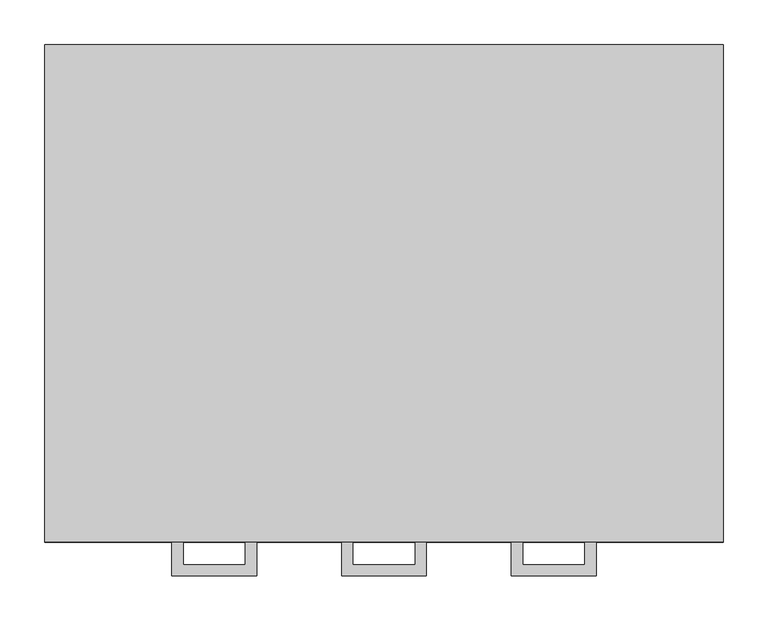
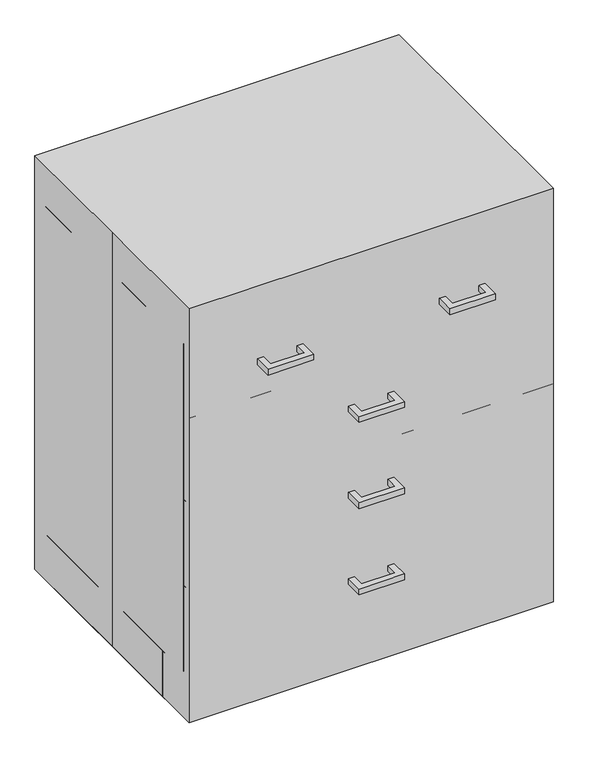
"""IFC4 building model written with IfcOpenShell, lengths in millimetres: proxy geometry, C03H0 - Cabinet, U-C-B, 2 Half DR, 3 DR, 36x30x22 : C03H0 - Cabinet, U-C-B, 2 Half DR, 3 DR, 36x30x22."""

from ifc_helpers import new_model, si_unit, frame, origin, origin_with_axes, place, context, project, spatial, polyline, outline, extrude, source, transform, mapped, element, save


def specialty_equipment_9ec7cdb3(model_context):
    return source(origin(), model_context, "Body", "SweptSolid", [
        extrude(outline(polyline([(-47.625, -317.5), (-47.625, -279.4), (-34.9409299, -279.4), (-34.9409299, -304.8159299), (34.9409299, -304.8159299), (34.9409299, -279.4), (47.625, -279.4), (47.625, -317.5), (-47.625, -317.5)])), frame((0.0, 0.0, 188.8962383), z_axis=(0.0, 0.0, 1.0), x_axis=(1.0, 0.0, 0.0)), (0.0, 0.0, 1.0), 12.7),
        extrude(outline(polyline([(-47.625, -317.5), (-47.625, -279.4), (-34.9409299, -279.4), (-34.9409299, -304.8159299), (34.9409299, -304.8159299), (34.9409299, -279.4), (47.625, -279.4), (47.625, -317.5), (-47.625, -317.5)])), frame((0.0, 0.0, 379.3962383), z_axis=(0.0, 0.0, 1.0), x_axis=(1.0, 0.0, 0.0)), (0.0, 0.0, 1.0), 12.7),
        extrude(outline(polyline([(-47.625, -317.5), (-47.625, -279.4), (-34.9409299, -279.4), (-34.9409299, -304.8159299), (34.9409299, -304.8159299), (34.9409299, -279.4), (47.625, -279.4), (47.625, -317.5), (-47.625, -317.5)])), frame((0.0, 0.0, 569.8962383), z_axis=(0.0, 0.0, 1.0), x_axis=(1.0, 0.0, 0.0)), (0.0, 0.0, 1.0), 12.7),
        extrude(outline(polyline([(-238.125, -317.5), (-238.125, -279.4), (-225.4409299, -279.4), (-225.4409299, -304.8159299), (-155.5590701, -304.8159299), (-155.5590701, -279.4), (-142.875, -279.4), (-142.875, -317.5), (-238.125, -317.5)])), frame((0.0, 0.0, 741.3462383), z_axis=(0.0, 0.0, 1.0), x_axis=(1.0, 0.0, 0.0)), (0.0, 0.0, 1.0), 12.7),
        extrude(outline(polyline([(238.125, -317.5), (142.875, -317.5), (142.875, -279.4), (155.5590701, -279.4), (155.5590701, -304.8159299), (225.4409299, -304.8159299), (225.4409299, -279.4), (238.125, -279.4), (238.125, -317.5)])), frame((0.0, 0.0, 741.3462383), z_axis=(0.0, 0.0, 1.0), x_axis=(1.0, 0.0, 0.0)), (0.0, 0.0, 1.0), 12.7),
        extrude(outline(polyline([(-381.0, 279.4), (381.0, 279.4), (381.0, -279.4), (-381.0, -279.4), (-381.0, 0.0), (-381.0, 279.4)])), origin_with_axes(), (0.0, 0.0, 1.0), 914.4),
        extrude(outline(polyline([(381.0, -279.4), (-381.0, -279.4), (-381.0, -260.35), (381.0, -260.35), (381.0, -279.4)])), frame((0.0, 0.0, 101.5674767), z_axis=(0.0, 0.0, 1.0), x_axis=(1.0, 0.0, 0.0)), (0.0, 0.0, 1.0), 190.5),
        extrude(outline(polyline([(381.0, -279.4), (-381.0, -279.4), (-381.0, -260.35), (381.0, -260.35), (381.0, -279.4)])), frame((0.0, 0.0, 292.0674767), z_axis=(0.0, 0.0, 1.0), x_axis=(1.0, 0.0, 0.0)), (0.0, 0.0, 1.0), 190.5),
        extrude(outline(polyline([(381.0, -279.4), (-381.0, -279.4), (-381.0, -260.35), (381.0, -260.35), (381.0, -279.4)])), frame((0.0, 0.0, 482.5674767), z_axis=(0.0, 0.0, 1.0), x_axis=(1.0, 0.0, 0.0)), (0.0, 0.0, 1.0), 190.5),
        extrude(outline(polyline([(381.0, -279.4), (0.0, -279.4), (0.0, -260.35), (381.0, -260.35), (381.0, -279.4)])), frame((0.0, 0.0, 673.0674767), z_axis=(0.0, 0.0, 1.0), x_axis=(1.0, 0.0, 0.0)), (0.0, 0.0, 1.0), 152.4),
        extrude(outline(polyline([(0.0, -279.4), (-381.0, -279.4), (-381.0, -260.35), (0.0, -260.35), (0.0, -279.4)])), frame((0.0, 0.0, 673.0674767), z_axis=(0.0, 0.0, 1.0), x_axis=(1.0, 0.0, 0.0)), (0.0, 0.0, 1.0), 152.4),
        extrude(outline(polyline([(-381.0, -260.35), (-381.0, 279.4), (-361.95, 279.4), (-361.95, -260.35), (-381.0, -260.35)])), frame((0.0, 0.0, 101.6), z_axis=(0.0, 0.0, 1.0), x_axis=(1.0, 0.0, 0.0)), (0.0, 0.0, 1.0), 723.8674767),
        extrude(outline(polyline([(361.95, -260.35), (361.95, 279.4), (381.0, 279.4), (381.0, -260.35), (361.95, -260.35)])), frame((0.0, 0.0, 101.6), z_axis=(0.0, 0.0, 1.0), x_axis=(1.0, 0.0, 0.0)), (0.0, 0.0, 1.0), 723.8674767),
        extrude(outline(polyline([(381.0, -203.2), (-381.0, -203.2), (-381.0, -184.15), (381.0, -184.15), (381.0, -203.2)])), origin_with_axes(), (0.0, 0.0, 1.0), 101.6),
        extrude(outline(polyline([(-381.0, -184.15), (-381.0, 279.4), (-361.95, 279.4), (-361.95, -184.15), (-381.0, -184.15)])), origin_with_axes(), (0.0, 0.0, 1.0), 101.6),
        extrude(outline(polyline([(361.95, -184.15), (361.95, 279.4), (381.0, 279.4), (381.0, -184.15), (361.95, -184.15)])), origin_with_axes(), (0.0, 0.0, 1.0), 101.6),
        extrude(outline(polyline([(381.0, 260.35), (-381.0, 260.35), (-381.0, 279.4), (381.0, 279.4), (381.0, 260.35)])), origin_with_axes(), (0.0, 0.0, 1.0), 101.6),
        extrude(outline(polyline([(361.95, 260.35), (361.95, -260.35), (-361.95, -260.35), (-361.95, 260.35), (361.95, 260.35)])), frame((0.0, 0.0, 101.6), z_axis=(0.0, 0.0, 1.0), x_axis=(1.0, 0.0, 0.0)), (0.0, 0.0, 1.0), 19.1166954),
        extrude(outline(polyline([(361.95, 260.35), (-361.95, 260.35), (-361.95, 279.4), (361.95, 279.4), (361.95, 260.35)])), frame((0.0, 0.0, 101.6), z_axis=(0.0, 0.0, 1.0), x_axis=(1.0, 0.0, 0.0)), (0.0, 0.0, 1.0), 704.8174767),
    ])


if __name__ == "__main__":
    model = new_model("IFC4")
    model_context = context("Model", 3, world=origin())
    ifc_project = project(units=[si_unit("LENGTHUNIT", "METRE", prefix="MILLI")], contexts=[model_context])
    site = spatial("IfcSite", under=ifc_project)
    building = spatial("IfcBuilding", under=site)
    placement = place(None, origin())
    specialty_equipment_shape = specialty_equipment_9ec7cdb3(model_context)
    element("IfcBuildingElementProxy", 1, Name="C03H0 - Cabinet, U-C-B, 2 Half DR, 3 DR, 36x30x22 : C03H0 - Cabinet, U-C-B, 2 Half DR, 3 DR, 36x30x22", ObjectType="C03H0 - Cabinet, U-C-B, 2 Half DR, 3 DR, 36x30x22 : C03H0 - Cabinet, U-C-B, 2 Half DR, 3 DR, 36x30x22", at=placement, inside=building, context=model_context, shape_type="MappedRepresentation", body=[
        mapped(specialty_equipment_shape, transform((0.0, 0.0, 0.0), x_axis=(1.0, 0.0, 0.0), y_axis=(0.0, 1.0, 0.0), z_axis=(0.0, 0.0, 1.0))),
    ])
    save(model, "model.ifc")

# Revit data of these elements
# Type "C03H0 - Cabinet, U-C-B, 2 Half DR, 3 DR, 36x30x22 : C03H0 - Cabinet, U-C-B, 2 Half DR, 3 DR, 36x30x22"
#   Watts2 = "0"
#   Watts1 = "0"
#   Unit_Issue = "EA"
#   UTIL_6_Misc = "-"
#   UTIL_5_NonMedGas = "-"
#   UTIL_4_MiscGas = "-"
#   UTIL_3_MedGas = "-"
#   UTIL_2_Elec = "-"
#   UTIL_1_WaterDrain = "-"
#   Nomenclature = "Cabinet, U/C/B, 1 Shelf, 2 Half DR, 2 DO, 36x30x22"
#   NSN = "6530"
#   Location [instance default] = ""
#   JSN = "C03H0"
#   Fund_Source_VA = "-"
#   Fund_Source_Navy = "-"
#   Fund_Source_Army = "-"
#   Fund_Source_AF = "-"
#   ELEC_Volts2 = "0"
#   ELEC_Volts1 = "0"
#   ELEC_Phase2 = "0"
#   ELEC_Phase1 = "0"
#   ELEC_HertzSwitch = "0"
#   ELEC_HertzDependent = "0"
#   ELEC_Hertz = "0"
#   ELEC_Amps2 = "0"
#   ELEC_Amps1 = "0"
#   DetailDescription = "Standing height under counter base cabinet with two half width drawers side-by-side above three full width drawers. Also referred to as a drawer cabinet. For general purpose use throughout the facility."
#   CAT_VA = "A"
#   CAT_Navy = "A"
#   CAT_IHS = "-"
#   CAT_Army = "A"
#   CAT_AF = "A"
#   BTUperhour = "0"
#   Weight_IP = 150
#   DIM_Width_IP = 2' - 6"
#   DIM_Height_IP = 3' - 0"
#   DIM_Depth_IP = 1' - 10"
#   Top Panel Material = none
#   Toe Panel Material = none
#   Side Panel Material = none
#   Shelf Panel Material = none
#   Drawer Front Material = none
#   Door Panel Material = none
#   Back Panel Material = none
#   Assembly Code = ""
# Element 1 (IfcBuildingElementProxy, "C03H0 - Cabinet, U-C-B, 2 Half DR, 3 DR, 36x30x22 : C03H0 - Cabinet, U-C-B, 2 Half DR, 3 DR, 36x30x22")
#   Materials on its faces: "Default metal", "EquipSpace"
# Materials
#   "Default metal": class "Unassigned", colour RGB 204 204 204, transparency 0
#   "EquipSpace": class "Unassigned", colour RGB 221 217 195, transparency 0.5
